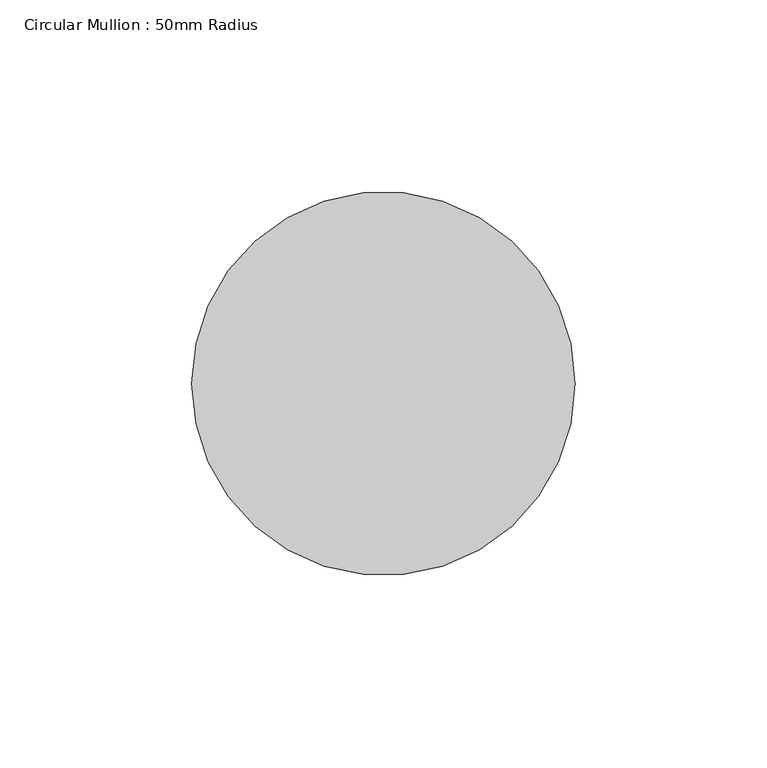
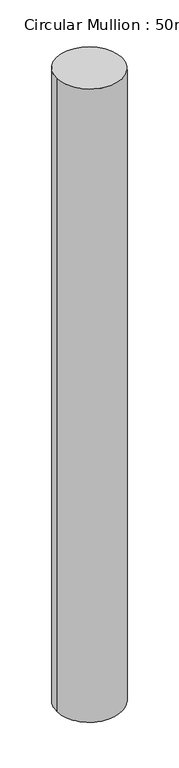
"""IFC4 building model written with IfcOpenShell, lengths in millimetres: member geometry, Circular Mullion : 50mm Radius."""

from ifc_helpers import new_model, si_unit, frame, origin, place, context, project, spatial, ellipse_curve, source, transform, mapped, element, save
from ifc_brep_helpers import plane_surface, cylinder_surface, advanced_brep


def circular_mullion_50mm_radius_e102a22f(model_context):
    return source(origin(), model_context, "Body", "AdvancedBrep", [
        advanced_brep(
        [(-100.0, 0.0, 1.5593508), (0.0, 0.0, 0.0), (0.0, 0.0, -1019.7174495), (-100.0, 0.0, -1021.2452147)],
        [
            (0, 1, ellipse_curve(frame((-50.0, 0.0, 0.7796754), z_axis=(-0.015589927276928098, -0.014703984727911667, -0.9997703471300904), x_axis=(-0.727307959145954, -0.6859765882036856, 0.021430188972067526)), 50.0114853, 50.0)),
            (1, 2),
            (2, 3, ellipse_curve(frame((-50.0, 0.0, -1020.4813321), z_axis=(-0.015274284536372697, -0.014406279295797918, 0.9997795533760199), x_axis=(0.7273146564599453, 0.6859829049235162, 0.02099630089434661)), 50.0110248, 50.0)),
            (3, 0),
            (1, 0, ellipse_curve(frame((-50.0, 0.0, 0.7796754), z_axis=(-0.015589927276928098, -0.014703984727911667, -0.9997703471300904), x_axis=(-0.727307959145954, -0.6859765882036856, 0.021430188972067526)), 50.0114853, 50.0)),
            (3, 2, ellipse_curve(frame((-50.0, 0.0, -1020.4813321), z_axis=(-0.015274284536372697, -0.014406279295797918, 0.9997795533760199), x_axis=(0.7273146564599453, 0.6859829049235162, 0.02099630089434661)), 50.0110248, 50.0)),
        ],
        [
            cylinder_surface(frame((-50.0, 0.0, 0.0), z_axis=(0.0, 0.0, 1.0), x_axis=(1.0, 0.0, 0.0)), 50.0),
            plane_surface(frame((-209.1336922, 221.7343879, 0.0), z_axis=(0.015589927276928102, 0.01470398472791167, 0.9997703471300906), x_axis=(0.7273079591459537, 0.685976588203686, -0.0214301889720685))),
            plane_surface(frame((-209.1336922, 221.7343879, -1019.7174495), z_axis=(0.015274284536372694, 0.014406279295797915, -0.9997795533760196), x_axis=(0.7273146564599451, 0.685982904923516, 0.020996300894362552))),
        ],
        [
            (0, [[1, 2, 3, 4]]),
            (0, [[5, -4, 6, -2]]),
            (1, [[-1, -5]]),
            (2, [[-6, -3]]),
        ],
    ),
    ])


if __name__ == "__main__":
    model = new_model("IFC4")
    model_context = context("Model", 3, world=origin())
    ifc_project = project(units=[si_unit("LENGTHUNIT", "METRE", prefix="MILLI")], contexts=[model_context])
    site = spatial("IfcSite", under=ifc_project)
    building = spatial("IfcBuilding", under=site)
    placement = place(None, origin())
    circular_mullion_50mm_radius_shape = circular_mullion_50mm_radius_e102a22f(model_context)
    element("IfcMember", 1, ObjectType="Circular Mullion : 50mm Radius", at=placement, inside=building, context=model_context, shape_type="MappedRepresentation", body=[
        mapped(circular_mullion_50mm_radius_shape, transform((0.0, 0.0, 0.0), x_axis=(1.0, 0.0, 0.0), y_axis=(0.0, 1.0, 0.0), z_axis=(0.0, 0.0, 1.0))),
    ])
    save(model, "model.ifc")

# Revit data of these elements
# Type "Circular Mullion : 50mm Radius"
#   built-in parameter 1007350 = 0.164042 (stored number, unit not read)
# Element 1 (IfcMember, "Circular Mullion : 50mm Radius")
#   Materials on its faces: "Aluminium"
# Materials
#   "Aluminium": class "Metal", colour RGB 247 247 247, transparency 0, Description = "Aluminium 6061", Cost = 0
